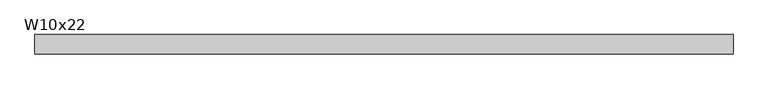
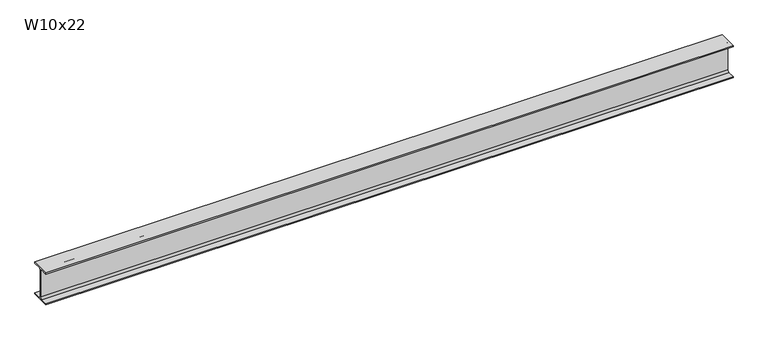
"""IFC4 building model written with IfcOpenShell, lengths in millimetres: beam geometry, RME W-Wide Flange : W10x22."""

import ifcopenshell
import ifcopenshell.guid

model = None  # the IFC model being written
_history = None  # IfcOwnerHistory: only IFC2X3 demands one
_inside = {}  # id of a spatial element -> (the spatial element, [elements in it])
_under = {}  # id of a project, library or spatial element -> (it, [spatial elements below it])
_declared = {}  # id of a project -> (the project, [libraries it declares])
_typed = {}  # id of a type object -> (the type object, [elements of that type])
_made_of = {}  # id of a material, layer set ... -> (it, [elements and type objects made of it])


def new_model(schema):
    """Start an empty IFC model of exactly this schema.

    Asked for "IFC4X3", IfcOpenShell would pick the latest addendum, in which some entities
    have other attributes; the version numbers below select the first issue.
    IFC2X3 requires an IfcOwnerHistory on every rooted entity: one is made here for all.
    """
    global model, _history
    if schema == "IFC4X3":
        model = ifcopenshell.file(schema_version=(4, 3, 0, 0))
    else:
        model = ifcopenshell.file(schema=schema)
    _inside.clear()
    _under.clear()
    _declared.clear()
    _typed.clear()
    _made_of.clear()
    _history = None
    if model.schema == "IFC2X3":
        org = make("IfcOrganization", Name="unknown")
        user = make(
            "IfcPersonAndOrganization",
            ThePerson=make("IfcPerson", FamilyName="unknown"),
            TheOrganization=org,
        )
        app = make(
            "IfcApplication",
            ApplicationDeveloper=org,
            Version="unknown",
            ApplicationFullName="unknown",
            ApplicationIdentifier="unknown",
        )
        _history = make(
            "IfcOwnerHistory",
            OwningUser=user,
            OwningApplication=app,
            ChangeAction="ADDED",
            CreationDate=0,
        )
    return model


def make(cls, **values):
    """One entity of the class cls with the attributes given. An attribute that is None is left unset."""
    return model.create_entity(
        cls, **{name: value for name, value in values.items() if value is not None}
    )


def rooted(cls, **values):
    """An entity with a GlobalId (a new one), such as an element, a storey or a relation."""
    return make(cls, GlobalId=ifcopenshell.guid.new(), OwnerHistory=_history, **values)


def si_unit(unit_type, name, prefix=None):
    """IfcSIUnit, for example si_unit("LENGTHUNIT", "METRE", prefix="MILLI")."""
    return make("IfcSIUnit", UnitType=unit_type, Prefix=prefix, Name=name)


def assignment(units):
    """IfcUnitAssignment: the units of a project."""
    return None if units is None else make("IfcUnitAssignment", Units=units)


def point(xyz):
    """IfcCartesianPoint."""
    return None if xyz is None else make("IfcCartesianPoint", Coordinates=xyz)


def direction(xyz):
    """IfcDirection."""
    return None if xyz is None else make("IfcDirection", DirectionRatios=xyz)


def frame(location, z_axis=None, x_axis=None):
    """IfcAxis2Placement3D, a coordinate frame: its origin and axes. An axis left out is left unset."""
    return make(
        "IfcAxis2Placement3D",
        Location=point(location),
        Axis=direction(z_axis),
        RefDirection=direction(x_axis),
    )


def frame_2d(location, x_axis=None):
    """IfcAxis2Placement2D, a coordinate frame in the plane: its origin and x axis."""
    return make(
        "IfcAxis2Placement2D", Location=point(location), RefDirection=direction(x_axis)
    )


def origin():
    """The frame at (0, 0, 0) with its axes left unset."""
    return frame((0.0, 0.0, 0.0))


def place(relative_to, where):
    """IfcLocalPlacement: puts the frame where relative to a parent placement (None: the world)."""
    return make(
        "IfcLocalPlacement", PlacementRelTo=relative_to, RelativePlacement=where
    )


def context(
    kind, dimensions, precision=None, world=None, true_north=None, identifier=None
):
    """IfcGeometricRepresentationContext, for example the 3D "Model" context."""
    return make(
        "IfcGeometricRepresentationContext",
        ContextIdentifier=identifier,
        ContextType=kind,
        CoordinateSpaceDimension=dimensions,
        Precision=precision,
        WorldCoordinateSystem=world,
        TrueNorth=true_north,
    )


def project(units=None, contexts=None):
    """IfcProject with its units and contexts."""
    return rooted(
        "IfcProject",
        Name="project",
        RepresentationContexts=contexts,
        UnitsInContext=assignment(units),
    )


def spatial(cls, under=None, at=None, **own):
    """A site, building, storey or space (cls), placed at a placement, below another one or the project."""
    s = rooted(cls, ObjectPlacement=at, **own)
    if under is not None:
        _under.setdefault(under.id(), (under, []))[1].append(s)
    return s


def polyline(points):
    """IfcPolyline through the points."""
    return make("IfcPolyline", Points=[point(p) for p in points])


def circle_curve(where, radius):
    """IfcCircle in the frame where."""
    return make("IfcCircle", Position=where, Radius=radius)


def trimmed(basis, trim1, trim2, sense, master):
    """IfcTrimmedCurve: the piece of a basis curve between two trims."""
    return make(
        "IfcTrimmedCurve",
        BasisCurve=basis,
        Trim1=trim1,
        Trim2=trim2,
        SenseAgreement=sense,
        MasterRepresentation=master,
    )


def segment(curve, same_sense, transition):
    """IfcCompositeCurveSegment."""
    return make(
        "IfcCompositeCurveSegment",
        Transition=transition,
        SameSense=same_sense,
        ParentCurve=curve,
    )


def composite_curve(segments, self_intersect=None):
    """IfcCompositeCurve: segments joined end to end."""
    return make("IfcCompositeCurve", Segments=segments, SelfIntersect=self_intersect)


def outline(outer, holes=None, kind="AREA"):
    """IfcArbitraryClosedProfileDef: a profile drawn as a closed curve; with holes, ...WithVoids."""
    if holes is None:
        return make("IfcArbitraryClosedProfileDef", ProfileType=kind, OuterCurve=outer)
    return make(
        "IfcArbitraryProfileDefWithVoids",
        ProfileType=kind,
        OuterCurve=outer,
        InnerCurves=holes,
    )


def extrude(swept, where, along, depth):
    """IfcExtrudedAreaSolid: the profile swept, set in the frame where, extruded along a direction by depth."""
    return make(
        "IfcExtrudedAreaSolid",
        SweptArea=swept,
        Position=where,
        ExtrudedDirection=direction(along),
        Depth=depth,
    )


def shape(context_of_items, identifier, shape_type, items):
    """IfcShapeRepresentation: the items that make up one representation, for example the "Body"."""
    return make(
        "IfcShapeRepresentation",
        ContextOfItems=context_of_items,
        RepresentationIdentifier=identifier,
        RepresentationType=shape_type,
        Items=items,
    )


def source(mapping_origin, context_of_items, identifier, shape_type, items):
    """IfcRepresentationMap: a shape defined once, which mapped items show again and again."""
    return make(
        "IfcRepresentationMap",
        MappingOrigin=mapping_origin,
        MappedRepresentation=shape(context_of_items, identifier, shape_type, items),
    )


def transform(
    local_origin,
    x_axis=None,
    y_axis=None,
    z_axis=None,
    scale=None,
    scale2=None,
    scale3=None,
    uniform=True,
):
    """IfcCartesianTransformationOperator3D, or its non-uniform kind. x_axis, y_axis, z_axis: its Axis1, 2, 3."""
    if uniform:
        return make(
            "IfcCartesianTransformationOperator3D",
            Axis1=direction(x_axis),
            Axis2=direction(y_axis),
            LocalOrigin=point(local_origin),
            Scale=scale,
            Axis3=direction(z_axis),
        )
    return make(
        "IfcCartesianTransformationOperator3DnonUniform",
        Axis1=direction(x_axis),
        Axis2=direction(y_axis),
        LocalOrigin=point(local_origin),
        Scale=scale,
        Axis3=direction(z_axis),
        Scale2=scale2,
        Scale3=scale3,
    )


def mapped(mapping_source, mapping_target):
    """IfcMappedItem: shows the shape of a source again, moved by a transform."""
    return make(
        "IfcMappedItem", MappingSource=mapping_source, MappingTarget=mapping_target
    )


def made_of(thing, what):
    """Note that an element or type object is made of a material, layer set ...; save() writes the relation."""
    if what is not None:
        _made_of.setdefault(what.id(), (what, []))[1].append(thing)
    return thing


def element(
    cls,
    number,
    at=None,
    inside=None,
    cuts=None,
    type_object=None,
    material=None,
    context=None,
    identifier="Body",
    shape_type=None,
    held_by="IfcProductDefinitionShape",
    body=None,
    shapes=None,
    **own,
):
    """One element of the class cls, such as IfcWall. Its Tag is "e" and its number.

    at: its placement. inside: the storey or other place that contains it. cuts: it is an
    opening in that element (IfcRelVoidsElement). A single representation is given by context,
    identifier, shape_type and body (its items); several are given by shapes. held_by: the class
    of the entity that holds the representations. save() writes the other relations.
    """
    e = rooted(cls, Tag="e%d" % number, ObjectPlacement=at, **own)
    if body is not None:
        shapes = [shape(context, identifier, shape_type, body)]
    if shapes is not None:
        e.Representation = make(held_by, Representations=shapes)
    if inside is not None:
        _inside.setdefault(inside.id(), (inside, []))[1].append(e)
    if cuts is not None:
        rooted(
            "IfcRelVoidsElement", RelatingBuildingElement=cuts, RelatedOpeningElement=e
        )
    if type_object is not None:
        _typed.setdefault(type_object.id(), (type_object, []))[1].append(e)
    return made_of(e, material)


def aggregate(whole, parts):
    """IfcRelAggregates: a whole, such as a stair, and the parts it consists of."""
    return rooted("IfcRelAggregates", RelatingObject=whole, RelatedObjects=parts)


def save(model, path):
    """Write the relations noted so far, then the file.

    IfcRelAggregates (storeys below a building ...), IfcRelContainedInSpatialStructure (elements
    in a storey), IfcRelDefinesByType, IfcRelAssociatesMaterial and IfcRelDeclares: one each for
    every whole, place, type object, material and project.
    """
    for whole, parts in _under.values():
        aggregate(whole, parts)
    for where, things in _inside.values():
        rooted(
            "IfcRelContainedInSpatialStructure",
            RelatedElements=things,
            RelatingStructure=where,
        )
    for kind, things in _typed.values():
        rooted("IfcRelDefinesByType", RelatedObjects=things, RelatingType=kind)
    for what, things in _made_of.values():
        rooted("IfcRelAssociatesMaterial", RelatedObjects=things, RelatingMaterial=what)
    for by, libraries in _declared.values():
        rooted("IfcRelDeclares", RelatingContext=by, RelatedDefinitions=libraries)
    model.write(path)


def w10x22_e5153db7(model_context):
    return source(origin(), model_context, "Body", "SweptSolid", [
        extrude(outline(composite_curve([segment(polyline([(73.025, -120.396), (73.025, -129.54), (-73.025, -129.54), (-73.025, -120.396), (-17.7165, -120.396)]), True, "CONTINUOUS"), segment(trimmed(circle_curve(frame_2d((-17.7165, -105.7275)), 14.6685), [point((-17.7165, -120.396))], [point((-3.048, -105.7275))], True, "CARTESIAN"), True, "CONTINUOUS"), segment(polyline([(-3.048, -105.7275), (-3.048, 105.7275)]), True, "CONTINUOUS"), segment(trimmed(circle_curve(frame_2d((-17.7165, 105.7275)), 14.6685), [point((-3.048, 105.7275))], [point((-17.7165, 120.396))], True, "CARTESIAN"), True, "CONTINUOUS"), segment(polyline([(-17.7165, 120.396), (-73.025, 120.396), (-73.025, 129.54), (73.025, 129.54), (73.025, 120.396), (17.7165, 120.396)]), True, "CONTINUOUS"), segment(trimmed(circle_curve(frame_2d((17.7165, 105.7275)), 14.6685), [point((17.7165, 120.396))], [point((3.048, 105.7275))], True, "CARTESIAN"), True, "CONTINUOUS"), segment(polyline([(3.048, 105.7275), (3.048, -105.7275)]), True, "CONTINUOUS"), segment(trimmed(circle_curve(frame_2d((17.7165, -105.7275)), 14.6685), [point((3.048, -105.7275))], [point((17.7165, -120.396))], True, "CARTESIAN"), True, "CONTINUOUS"), segment(polyline([(17.7165, -120.396), (73.025, -120.396)]), True, "CONTINUOUS")], self_intersect=False)), frame((-2628.9, 0.0, 0.0), z_axis=(1.0, 0.0, 0.0), x_axis=(0.0, 1.0, 0.0)), (0.0, 0.0, 1.0), 5257.8),
    ])


if __name__ == "__main__":
    model = new_model("IFC4")
    model_context = context("Model", 3, world=origin())
    ifc_project = project(units=[si_unit("LENGTHUNIT", "METRE", prefix="MILLI")], contexts=[model_context])
    site = spatial("IfcSite", under=ifc_project)
    building = spatial("IfcBuilding", under=site)
    placement = place(None, origin())
    w10x22_shape = w10x22_e5153db7(model_context)
    element("IfcBeam", 1, ObjectType="RME W-Wide Flange : W10x22", at=placement, inside=building, context=model_context, shape_type="MappedRepresentation", body=[
        mapped(w10x22_shape, transform((0.0, 0.0, 0.0), x_axis=(1.0, 0.0, 0.0), y_axis=(0.0, 1.0, 0.0), z_axis=(0.0, 0.0, 1.0))),
    ])
    save(model, "model.ifc")

# Revit data of these elements
# Type "RME W-Wide Flange : W10x22"
#   WELD P [instance default] = ""
#   WELD LE [instance default] = ""
#   WELD D [instance default] = ""
#   TOP SECTION SIZE [instance default] = ""
#   TOP SECTION LENGTH [instance default] = ""
#   REMARKS [instance default] = ""
#   REINF TYPE [instance default] = ""
#   Nominal Size = "W24"
#   End Bearing Capacity [instance default] = ""
#   BOT SECTION SIZE [instance default] = ""
#   BOT SECTION LENGTH [instance default] = ""
#   Assembly Code = "B10"
#   W = 22
#   Start Extension Calculation [instance default] = 10' - 0"
#   Start Extension [instance default] = -0' - 0 1/2"
#   End Extension Calculation [instance default] = 10' - 0"
#   End Extension [instance default] = -0' - 0 1/2"
#   Length [instance default] = 5' - 0"
#   bf = 0' - 5 3/4"
#   d = 0' - 10.2"
#   k = 0' - 0 15/16"
#   k2 = 0' - 0.5775"
#   tf = 0' - 0.36"
#   tw = 0' - 0.24"
#   A = 0.0450694 SF
#   Structural Material [instance default] = Metal - Steel - ASTM A992
# Element 1 (IfcBeam, "RME W-Wide Flange : W10x22")
#   Length = 17' - 3"
#   Materials on its faces: "Metal - Steel - ASTM A992"
# Materials
#   "Metal - Steel - ASTM A992": class "Metal", colour RGB 255 128 0, transparency 0
